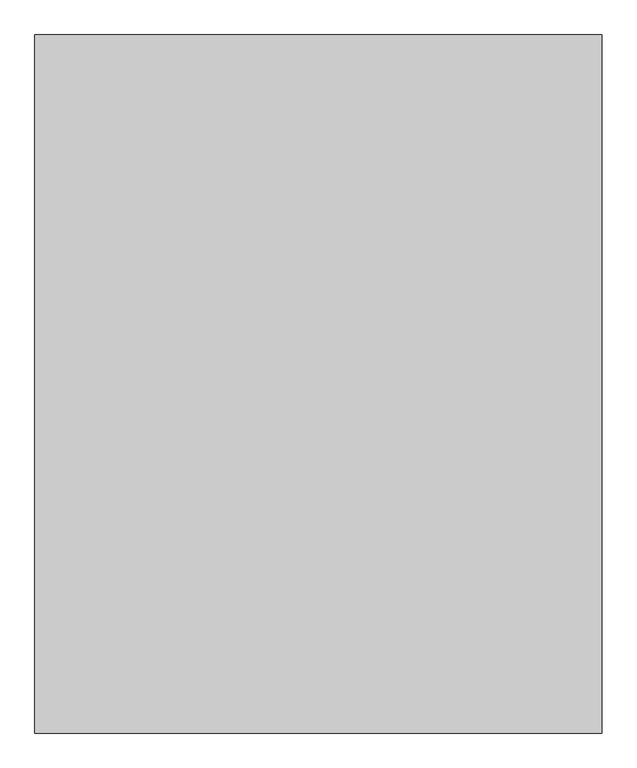
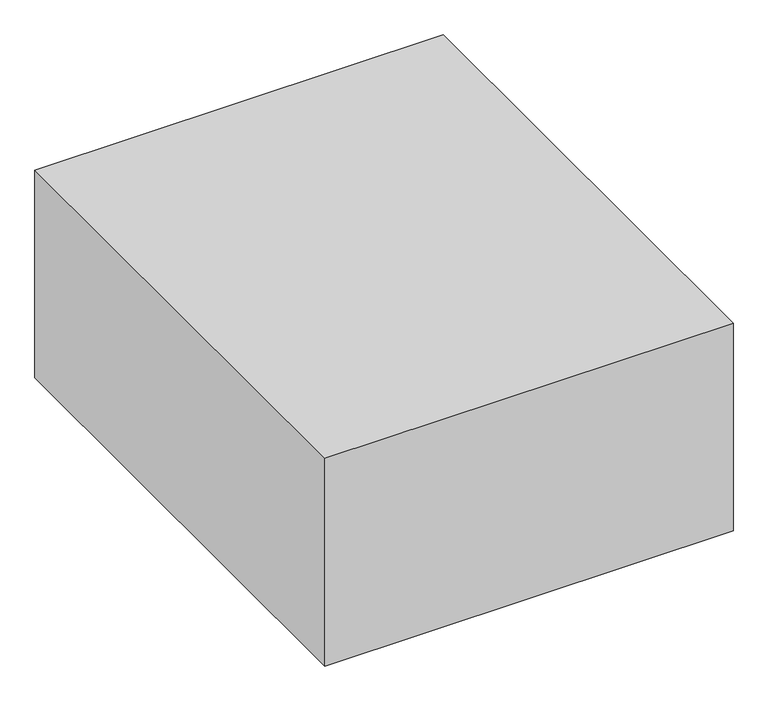
"""IFC4 building model written with IfcOpenShell, lengths in millimetres: proxy geometry, Space Planning Box_hec : Space Planning Box_hec."""

import ifcopenshell
import ifcopenshell.guid

model = None  # the IFC model being written
_history = None  # IfcOwnerHistory: only IFC2X3 demands one
_inside = {}  # id of a spatial element -> (the spatial element, [elements in it])
_under = {}  # id of a project, library or spatial element -> (it, [spatial elements below it])
_declared = {}  # id of a project -> (the project, [libraries it declares])
_typed = {}  # id of a type object -> (the type object, [elements of that type])
_made_of = {}  # id of a material, layer set ... -> (it, [elements and type objects made of it])


def new_model(schema):
    """Start an empty IFC model of exactly this schema.

    Asked for "IFC4X3", IfcOpenShell would pick the latest addendum, in which some entities
    have other attributes; the version numbers below select the first issue.
    IFC2X3 requires an IfcOwnerHistory on every rooted entity: one is made here for all.
    """
    global model, _history
    if schema == "IFC4X3":
        model = ifcopenshell.file(schema_version=(4, 3, 0, 0))
    else:
        model = ifcopenshell.file(schema=schema)
    _inside.clear()
    _under.clear()
    _declared.clear()
    _typed.clear()
    _made_of.clear()
    _history = None
    if model.schema == "IFC2X3":
        org = make("IfcOrganization", Name="unknown")
        user = make(
            "IfcPersonAndOrganization",
            ThePerson=make("IfcPerson", FamilyName="unknown"),
            TheOrganization=org,
        )
        app = make(
            "IfcApplication",
            ApplicationDeveloper=org,
            Version="unknown",
            ApplicationFullName="unknown",
            ApplicationIdentifier="unknown",
        )
        _history = make(
            "IfcOwnerHistory",
            OwningUser=user,
            OwningApplication=app,
            ChangeAction="ADDED",
            CreationDate=0,
        )
    return model


def make(cls, **values):
    """One entity of the class cls with the attributes given. An attribute that is None is left unset."""
    return model.create_entity(
        cls, **{name: value for name, value in values.items() if value is not None}
    )


def rooted(cls, **values):
    """An entity with a GlobalId (a new one), such as an element, a storey or a relation."""
    return make(cls, GlobalId=ifcopenshell.guid.new(), OwnerHistory=_history, **values)


def si_unit(unit_type, name, prefix=None):
    """IfcSIUnit, for example si_unit("LENGTHUNIT", "METRE", prefix="MILLI")."""
    return make("IfcSIUnit", UnitType=unit_type, Prefix=prefix, Name=name)


def assignment(units):
    """IfcUnitAssignment: the units of a project."""
    return None if units is None else make("IfcUnitAssignment", Units=units)


def point(xyz):
    """IfcCartesianPoint."""
    return None if xyz is None else make("IfcCartesianPoint", Coordinates=xyz)


def direction(xyz):
    """IfcDirection."""
    return None if xyz is None else make("IfcDirection", DirectionRatios=xyz)


def frame(location, z_axis=None, x_axis=None):
    """IfcAxis2Placement3D, a coordinate frame: its origin and axes. An axis left out is left unset."""
    return make(
        "IfcAxis2Placement3D",
        Location=point(location),
        Axis=direction(z_axis),
        RefDirection=direction(x_axis),
    )


def origin():
    """The frame at (0, 0, 0) with its axes left unset."""
    return frame((0.0, 0.0, 0.0))


def origin_with_axes():
    """The frame at (0, 0, 0) with the z axis (0, 0, 1) and the x axis (1, 0, 0) written out."""
    return frame((0.0, 0.0, 0.0), z_axis=(0.0, 0.0, 1.0), x_axis=(1.0, 0.0, 0.0))


def place(relative_to, where):
    """IfcLocalPlacement: puts the frame where relative to a parent placement (None: the world)."""
    return make(
        "IfcLocalPlacement", PlacementRelTo=relative_to, RelativePlacement=where
    )


def context(
    kind, dimensions, precision=None, world=None, true_north=None, identifier=None
):
    """IfcGeometricRepresentationContext, for example the 3D "Model" context."""
    return make(
        "IfcGeometricRepresentationContext",
        ContextIdentifier=identifier,
        ContextType=kind,
        CoordinateSpaceDimension=dimensions,
        Precision=precision,
        WorldCoordinateSystem=world,
        TrueNorth=true_north,
    )


def project(units=None, contexts=None):
    """IfcProject with its units and contexts."""
    return rooted(
        "IfcProject",
        Name="project",
        RepresentationContexts=contexts,
        UnitsInContext=assignment(units),
    )


def spatial(cls, under=None, at=None, **own):
    """A site, building, storey or space (cls), placed at a placement, below another one or the project."""
    s = rooted(cls, ObjectPlacement=at, **own)
    if under is not None:
        _under.setdefault(under.id(), (under, []))[1].append(s)
    return s


def polyline(points):
    """IfcPolyline through the points."""
    return make("IfcPolyline", Points=[point(p) for p in points])


def outline(outer, holes=None, kind="AREA"):
    """IfcArbitraryClosedProfileDef: a profile drawn as a closed curve; with holes, ...WithVoids."""
    if holes is None:
        return make("IfcArbitraryClosedProfileDef", ProfileType=kind, OuterCurve=outer)
    return make(
        "IfcArbitraryProfileDefWithVoids",
        ProfileType=kind,
        OuterCurve=outer,
        InnerCurves=holes,
    )


def extrude(swept, where, along, depth):
    """IfcExtrudedAreaSolid: the profile swept, set in the frame where, extruded along a direction by depth."""
    return make(
        "IfcExtrudedAreaSolid",
        SweptArea=swept,
        Position=where,
        ExtrudedDirection=direction(along),
        Depth=depth,
    )


def shape(context_of_items, identifier, shape_type, items):
    """IfcShapeRepresentation: the items that make up one representation, for example the "Body"."""
    return make(
        "IfcShapeRepresentation",
        ContextOfItems=context_of_items,
        RepresentationIdentifier=identifier,
        RepresentationType=shape_type,
        Items=items,
    )


def source(mapping_origin, context_of_items, identifier, shape_type, items):
    """IfcRepresentationMap: a shape defined once, which mapped items show again and again."""
    return make(
        "IfcRepresentationMap",
        MappingOrigin=mapping_origin,
        MappedRepresentation=shape(context_of_items, identifier, shape_type, items),
    )


def transform(
    local_origin,
    x_axis=None,
    y_axis=None,
    z_axis=None,
    scale=None,
    scale2=None,
    scale3=None,
    uniform=True,
):
    """IfcCartesianTransformationOperator3D, or its non-uniform kind. x_axis, y_axis, z_axis: its Axis1, 2, 3."""
    if uniform:
        return make(
            "IfcCartesianTransformationOperator3D",
            Axis1=direction(x_axis),
            Axis2=direction(y_axis),
            LocalOrigin=point(local_origin),
            Scale=scale,
            Axis3=direction(z_axis),
        )
    return make(
        "IfcCartesianTransformationOperator3DnonUniform",
        Axis1=direction(x_axis),
        Axis2=direction(y_axis),
        LocalOrigin=point(local_origin),
        Scale=scale,
        Axis3=direction(z_axis),
        Scale2=scale2,
        Scale3=scale3,
    )


def mapped(mapping_source, mapping_target):
    """IfcMappedItem: shows the shape of a source again, moved by a transform."""
    return make(
        "IfcMappedItem", MappingSource=mapping_source, MappingTarget=mapping_target
    )


def made_of(thing, what):
    """Note that an element or type object is made of a material, layer set ...; save() writes the relation."""
    if what is not None:
        _made_of.setdefault(what.id(), (what, []))[1].append(thing)
    return thing


def element(
    cls,
    number,
    at=None,
    inside=None,
    cuts=None,
    type_object=None,
    material=None,
    context=None,
    identifier="Body",
    shape_type=None,
    held_by="IfcProductDefinitionShape",
    body=None,
    shapes=None,
    **own,
):
    """One element of the class cls, such as IfcWall. Its Tag is "e" and its number.

    at: its placement. inside: the storey or other place that contains it. cuts: it is an
    opening in that element (IfcRelVoidsElement). A single representation is given by context,
    identifier, shape_type and body (its items); several are given by shapes. held_by: the class
    of the entity that holds the representations. save() writes the other relations.
    """
    e = rooted(cls, Tag="e%d" % number, ObjectPlacement=at, **own)
    if body is not None:
        shapes = [shape(context, identifier, shape_type, body)]
    if shapes is not None:
        e.Representation = make(held_by, Representations=shapes)
    if inside is not None:
        _inside.setdefault(inside.id(), (inside, []))[1].append(e)
    if cuts is not None:
        rooted(
            "IfcRelVoidsElement", RelatingBuildingElement=cuts, RelatedOpeningElement=e
        )
    if type_object is not None:
        _typed.setdefault(type_object.id(), (type_object, []))[1].append(e)
    return made_of(e, material)


def aggregate(whole, parts):
    """IfcRelAggregates: a whole, such as a stair, and the parts it consists of."""
    return rooted("IfcRelAggregates", RelatingObject=whole, RelatedObjects=parts)


def save(model, path):
    """Write the relations noted so far, then the file.

    IfcRelAggregates (storeys below a building ...), IfcRelContainedInSpatialStructure (elements
    in a storey), IfcRelDefinesByType, IfcRelAssociatesMaterial and IfcRelDeclares: one each for
    every whole, place, type object, material and project.
    """
    for whole, parts in _under.values():
        aggregate(whole, parts)
    for where, things in _inside.values():
        rooted(
            "IfcRelContainedInSpatialStructure",
            RelatedElements=things,
            RelatingStructure=where,
        )
    for kind, things in _typed.values():
        rooted("IfcRelDefinesByType", RelatedObjects=things, RelatingType=kind)
    for what, things in _made_of.values():
        rooted("IfcRelAssociatesMaterial", RelatedObjects=things, RelatingMaterial=what)
    for by, libraries in _declared.values():
        rooted("IfcRelDeclares", RelatingContext=by, RelatedDefinitions=libraries)
    model.write(path)


def generic_models_70f6ae48(model_context):
    return source(origin(), model_context, "Body", "SweptSolid", [
        extrude(outline(polyline([(3250.0, 4000.0), (3250.0, -4000.0), (-3250.0, -4000.0), (-3250.0, 4000.0), (3250.0, 4000.0)])), origin_with_axes(), (0.0, 0.0, 1.0), 3500.0),
    ])


if __name__ == "__main__":
    model = new_model("IFC4")
    model_context = context("Model", 3, world=origin())
    ifc_project = project(units=[si_unit("LENGTHUNIT", "METRE", prefix="MILLI")], contexts=[model_context])
    site = spatial("IfcSite", under=ifc_project)
    building = spatial("IfcBuilding", under=site)
    placement = place(None, origin())
    generic_models_shape = generic_models_70f6ae48(model_context)
    element("IfcBuildingElementProxy", 1, Name="Space Planning Box_hec : Space Planning Box_hec", ObjectType="Space Planning Box_hec : Space Planning Box_hec", at=placement, inside=building, context=model_context, shape_type="MappedRepresentation", body=[
        mapped(generic_models_shape, transform((0.0, 0.0, 0.0), x_axis=(1.0, 0.0, 0.0), y_axis=(0.0, 1.0, 0.0), z_axis=(0.0, 0.0, 1.0))),
    ])
    save(model, "model.ifc")

# Revit data of these elements
# Type "Space Planning Box_hec : Space Planning Box_hec"
#   Type Comments = "..."
#   Room Name [instance default] = "?"
#   Interior Finish [instance default] = ""
#   Exterior Finish [instance default] = ""
#   Department [instance default] = ""
#   Assembly Code = "..."
#   ceiling height [instance default] = 0
#   Width [instance default] = 1524 mm
#   Program Area [instance default] = 0.00 m²
#   Length [instance default] = 1524 mm
#   Height [instance default] = 1524 mm
#   Area [instance default] = 2.32258 m²
#   Fill Color [instance default] = Cyan
#   Default Elevation = 0
# Element 1 (IfcBuildingElementProxy, "Space Planning Box_hec : Space Planning Box_hec")
#   Room Name = "Meeting Room-2"
#   Exterior Finish = "RF1..N/A,,EW1..N/A..N/A"
#   Department = "AR"
#   Width = 6500 mm
#   Program Area = 52.00 m²
#   Length = 8000 mm
#   Height = 3500 mm
#   Area = 52.00 m²
#   Materials on its faces: "Cyan"
# Materials
#   "Cyan": class "Generic", colour RGB 0 255 255, transparency 0.2, Cost = 0
